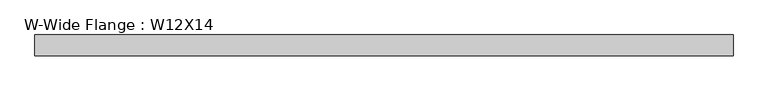
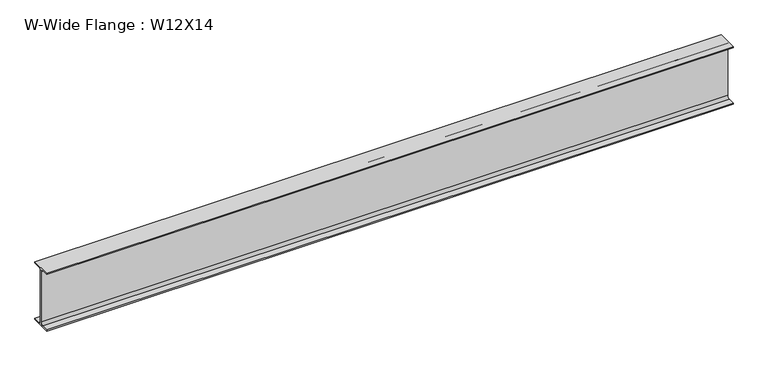
"""IFC4 building model written with IfcOpenShell, lengths in millimetres: beam geometry, W-Wide Flange : W12X14."""

from ifc_helpers import new_model, si_unit, point, frame, frame_2d, origin, place, context, project, spatial, polyline, circle_curve, trimmed, segment, composite_curve, outline, extrude, source, transform, mapped, element, save


def w_wide_flange_w12x14_42b2b6c6(model_context):
    return source(origin(), model_context, "Body", "SweptSolid", [
        extrude(outline(composite_curve([segment(polyline([(50.419, -145.415), (50.419, -151.13), (-50.419, -151.13), (-50.419, -145.415), (-15.875, -145.415)]), True, "CONTINUOUS"), segment(trimmed(circle_curve(frame_2d((-15.875, -132.08)), 13.335), [point((-15.875, -145.415))], [point((-2.54, -132.08))], True, "CARTESIAN"), True, "CONTINUOUS"), segment(polyline([(-2.54, -132.08), (-2.54, 132.08)]), True, "CONTINUOUS"), segment(trimmed(circle_curve(frame_2d((-15.875, 132.08)), 13.335), [point((-2.54, 132.08))], [point((-15.875, 145.415))], True, "CARTESIAN"), True, "CONTINUOUS"), segment(polyline([(-15.875, 145.415), (-50.419, 145.415), (-50.419, 151.13), (50.419, 151.13), (50.419, 145.415), (15.875, 145.415)]), True, "CONTINUOUS"), segment(trimmed(circle_curve(frame_2d((15.875, 132.08)), 13.335), [point((15.875, 145.415))], [point((2.54, 132.08))], True, "CARTESIAN"), True, "CONTINUOUS"), segment(polyline([(2.54, 132.08), (2.54, -132.08)]), True, "CONTINUOUS"), segment(trimmed(circle_curve(frame_2d((15.875, -132.08)), 13.335), [point((2.54, -132.08))], [point((15.875, -145.415))], True, "CARTESIAN"), True, "CONTINUOUS"), segment(polyline([(15.875, -145.415), (50.419, -145.415)]), True, "CONTINUOUS")], self_intersect=False)), frame((-1701.7761875, 0.0, 0.0), z_axis=(1.0, 0.0, 0.0), x_axis=(0.0, 1.0, 0.0)), (0.0, 0.0, 1.0), 3403.552375),
    ])


if __name__ == "__main__":
    model = new_model("IFC4")
    model_context = context("Model", 3, world=origin())
    ifc_project = project(units=[si_unit("LENGTHUNIT", "METRE", prefix="MILLI")], contexts=[model_context])
    site = spatial("IfcSite", under=ifc_project)
    building = spatial("IfcBuilding", under=site)
    placement = place(None, origin())
    w_wide_flange_w12x14_shape = w_wide_flange_w12x14_42b2b6c6(model_context)
    element("IfcBeam", 1, ObjectType="W-Wide Flange : W12X14", at=placement, inside=building, context=model_context, shape_type="MappedRepresentation", body=[
        mapped(w_wide_flange_w12x14_shape, transform((0.0, 0.0, 0.0), x_axis=(1.0, 0.0, 0.0), y_axis=(0.0, 1.0, 0.0), z_axis=(0.0, 0.0, 1.0))),
    ])
    save(model, "model.ifc")

# Revit data of these elements
# Type "W-Wide Flange : W12X14"
#   Assembly Code = "B10"
#   W = 14
#   Length [instance default] = 5' - 0"
#   bf = 0' - 3.97"
#   d = 0' - 11.9"
#   k = 0' - 0 3/4"
#   k2 = 0' - 0.525"
#   tf = 0' - 0.225"
#   tw = 0' - 0.2"
#   A = 0.0288889 SF
#   Structural Material [instance default] = Steel ASTM A992
# Element 1 (IfcBeam, "W-Wide Flange : W12X14")
#   Materials on its faces: "Steel ASTM A992"
# Materials
#   "Steel ASTM A992": class "Metal", colour RGB 199 199 199, transparency 0, Description = "Structural steel 50ksi", Cost = 0
